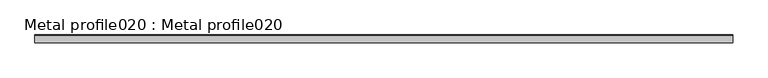
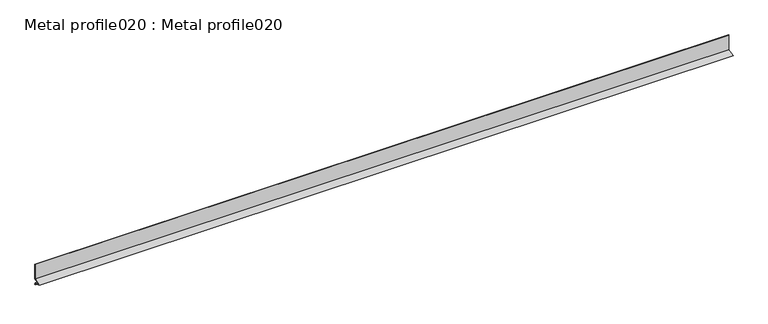
"""IFC4 building model written with IfcOpenShell, lengths in millimetres: proxy geometry, Metal profile020 : Metal profile020."""

from ifc_helpers import new_model, si_unit, frame, origin, place, context, project, spatial, polyline, outline, extrude, source, transform, mapped, element, save


def metal_profile020_metal_profile020_bf09e292(model_context):
    return source(origin(), model_context, "Body", "SweptSolid", [
        extrude(outline(polyline([(-4412.1175368, 40296.1778532), (-4413.3655993, 40295.9428216), (-4414.1889203, 40300.3148134), (-4434.3425368, 40306.7927615), (-4413.3875368, 40313.5282972), (-4413.3875368, 40357.5927615), (-4412.1175368, 40357.5927615), (-4412.1175368, 40312.6025179), (-4430.1923345, 40306.7927615), (-4413.0807319, 40301.2926035), (-4412.1175368, 40296.1778532)])), frame((12383.0178845, 0.0, 0.0), z_axis=(1.0, 0.0, 0.0), x_axis=(0.0, 1.0, 0.0)), (0.0, 0.0, 1.0), 2000.0),
    ])


if __name__ == "__main__":
    model = new_model("IFC4")
    model_context = context("Model", 3, world=origin())
    ifc_project = project(units=[si_unit("LENGTHUNIT", "METRE", prefix="MILLI")], contexts=[model_context])
    site = spatial("IfcSite", under=ifc_project)
    building = spatial("IfcBuilding", under=site)
    placement = place(None, origin())
    metal_profile020_metal_profile020_shape = metal_profile020_metal_profile020_bf09e292(model_context)
    element("IfcBuildingElementProxy", 1, Name="Metal profile020 : Metal profile020", ObjectType="Metal profile020 : Metal profile020", at=placement, inside=building, context=model_context, shape_type="MappedRepresentation", body=[
        mapped(metal_profile020_metal_profile020_shape, transform((0.0, 0.0, 0.0), x_axis=(1.0, 0.0, 0.0), y_axis=(0.0, 1.0, 0.0), z_axis=(0.0, 0.0, 1.0))),
    ])
    save(model, "model.ifc")

# Revit data of these elements
# Type "Metal profile020 : Metal profile020"
#   NameOverride = "Metal profile020"
# Element 1 (IfcBuildingElementProxy, "Metal profile020 : Metal profile020")
#   Materials on its faces: "16 GA. COPPER WEEP SCREED W/ MIN 3 1/2\" ATTACHMENT FLANGE - LAP UNDERLAYMENT OVER WEED SCREED"
# Materials
#   "16 GA. COPPER WEEP SCREED W/ MIN 3 1/2\" ATTACHMENT FLANGE - LAP UNDERLAYMENT OVER WEED SCREED": class "Unassigned", colour RGB 255 237 20, transparency 0
